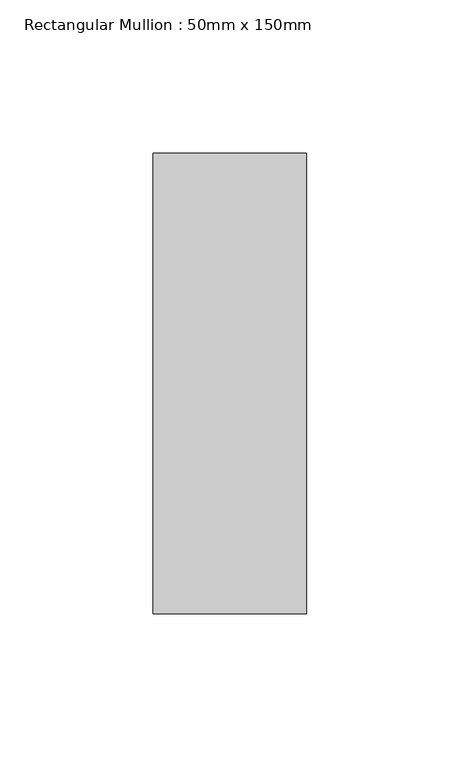
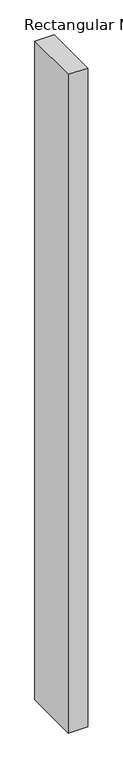
"""IFC4 building model written with IfcOpenShell, lengths in millimetres: member geometry, Rectangular Mullion : 50mm x 150mm."""

from ifc_helpers import new_model, si_unit, frame, origin, place, context, project, spatial, polyline, outline, extrude, source, transform, mapped, element, save


def rectangular_mullion_50mm_x_150mm_2da73195(model_context):
    return source(origin(), model_context, "Body", "SweptSolid", [
        extrude(outline(polyline([(0.0, 75.0), (0.0, -75.0), (-50.0, -75.0), (-50.0, 75.0), (0.0, 75.0)])), frame((0.0, 0.0, -1805.0000003), z_axis=(0.0, 0.0, 1.0), x_axis=(1.0, 0.0, 0.0)), (0.0, 0.0, 1.0), 1805.0000003),
    ])


if __name__ == "__main__":
    model = new_model("IFC4")
    model_context = context("Model", 3, world=origin())
    ifc_project = project(units=[si_unit("LENGTHUNIT", "METRE", prefix="MILLI")], contexts=[model_context])
    site = spatial("IfcSite", under=ifc_project)
    building = spatial("IfcBuilding", under=site)
    placement = place(None, origin())
    rectangular_mullion_50mm_x_150mm_shape = rectangular_mullion_50mm_x_150mm_2da73195(model_context)
    element("IfcMember", 1, ObjectType="Rectangular Mullion : 50mm x 150mm", at=placement, inside=building, context=model_context, shape_type="MappedRepresentation", body=[
        mapped(rectangular_mullion_50mm_x_150mm_shape, transform((0.0, 0.0, 0.0), x_axis=(1.0, 0.0, 0.0), y_axis=(0.0, 1.0, 0.0), z_axis=(0.0, 0.0, 1.0))),
    ])
    save(model, "model.ifc")

# Revit data of these elements
# Type "Rectangular Mullion : 50mm x 150mm"
#   built-in parameter 1007304 = 0.492126 (stored number, unit not read)
#   built-in parameter 1007301 = 0.082021 (stored number, unit not read)
#   built-in parameter 1007300 = 0.082021 (stored number, unit not read)
# Element 1 (IfcMember, "Rectangular Mullion : 50mm x 150mm")
#   Materials on its faces: "Aluminum"
# Materials
#   "Aluminum": class "Metal", colour RGB 244 244 244, transparency 0, Description = "Aluminum 6061", Cost = 0
